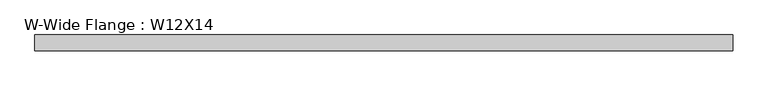
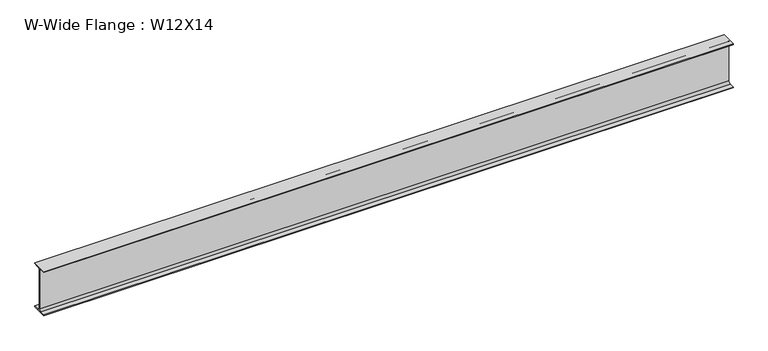
"""IFC4 building model written with IfcOpenShell, lengths in millimetres: beam geometry, W-Wide Flange : W12X14."""

from ifc_helpers import new_model, si_unit, point, frame, frame_2d, origin, place, context, project, spatial, polyline, circle_curve, trimmed, segment, composite_curve, outline, extrude, source, transform, mapped, element, save


def w_wide_flange_w12x14_677513c1(model_context):
    return source(origin(), model_context, "Body", "SweptSolid", [
        extrude(outline(composite_curve([segment(polyline([(50.419, -145.415), (50.419, -151.13), (-50.419, -151.13), (-50.419, -145.415), (-15.875, -145.415)]), True, "CONTINUOUS"), segment(trimmed(circle_curve(frame_2d((-15.875, -132.08)), 13.335), [point((-15.875, -145.415))], [point((-2.54, -132.08))], True, "CARTESIAN"), True, "CONTINUOUS"), segment(polyline([(-2.54, -132.08), (-2.54, 132.08)]), True, "CONTINUOUS"), segment(trimmed(circle_curve(frame_2d((-15.875, 132.08)), 13.335), [point((-2.54, 132.08))], [point((-15.875, 145.415))], True, "CARTESIAN"), True, "CONTINUOUS"), segment(polyline([(-15.875, 145.415), (-50.419, 145.415), (-50.419, 151.13), (50.419, 151.13), (50.419, 145.415), (15.875, 145.415)]), True, "CONTINUOUS"), segment(trimmed(circle_curve(frame_2d((15.875, 132.08)), 13.335), [point((15.875, 145.415))], [point((2.54, 132.08))], True, "CARTESIAN"), True, "CONTINUOUS"), segment(polyline([(2.54, 132.08), (2.54, -132.08)]), True, "CONTINUOUS"), segment(trimmed(circle_curve(frame_2d((15.875, -132.08)), 13.335), [point((2.54, -132.08))], [point((15.875, -145.415))], True, "CARTESIAN"), True, "CONTINUOUS"), segment(polyline([(15.875, -145.415), (50.419, -145.415)]), True, "CONTINUOUS")], self_intersect=False)), frame((-2235.2, 0.0, 0.0), z_axis=(1.0, 0.0, 0.0), x_axis=(0.0, 1.0, 0.0)), (0.0, 0.0, 1.0), 4470.146),
    ])


if __name__ == "__main__":
    model = new_model("IFC4")
    model_context = context("Model", 3, world=origin())
    ifc_project = project(units=[si_unit("LENGTHUNIT", "METRE", prefix="MILLI")], contexts=[model_context])
    site = spatial("IfcSite", under=ifc_project)
    building = spatial("IfcBuilding", under=site)
    placement = place(None, origin())
    w_wide_flange_w12x14_shape = w_wide_flange_w12x14_677513c1(model_context)
    element("IfcBeam", 1, ObjectType="W-Wide Flange : W12X14", at=placement, inside=building, context=model_context, shape_type="MappedRepresentation", body=[
        mapped(w_wide_flange_w12x14_shape, transform((0.0, 0.0, 0.0), x_axis=(1.0, 0.0, 0.0), y_axis=(0.0, 1.0, 0.0), z_axis=(0.0, 0.0, 1.0))),
    ])
    save(model, "model.ifc")

# Revit data of these elements
# Type "W-Wide Flange : W12X14"
#   Assembly Code = "B10"
#   W = 14
#   Length [instance default] = 5' - 0"
#   bf = 0' - 3.97"
#   d = 0' - 11.9"
#   k = 0' - 0 3/4"
#   k2 = 0' - 0.525"
#   tf = 0' - 0.225"
#   tw = 0' - 0.2"
#   A = 0.0288889 SF
#   Structural Material [instance default] = Steel ASTM A992
# Element 1 (IfcBeam, "W-Wide Flange : W12X14")
#   Materials on its faces: "Steel ASTM A992"
# Materials
#   "Steel ASTM A992": class "Metal", colour RGB 199 199 199, transparency 0, Description = "Structural steel 50ksi", Cost = 0
